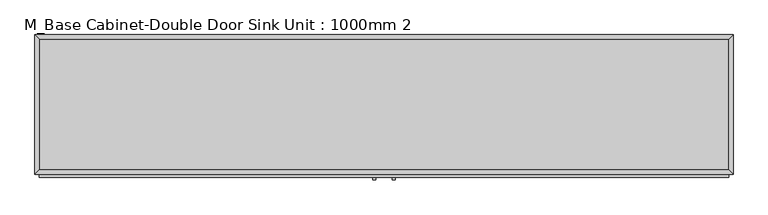
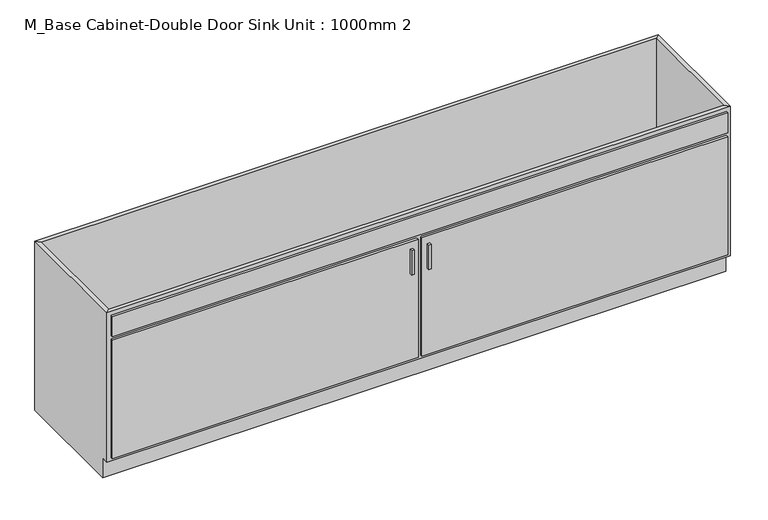
"""IFC4 building model written with IfcOpenShell, lengths in millimetres: furniture geometry, M_Base Cabinet-Double Door Sink Unit : 1000mm 2."""

from ifc_helpers import new_model, si_unit, frame, origin, place, context, project, spatial, polyline, outline, extrude, faceted_brep, source, transform, mapped, element, save


def m_base_cabinet_double_door_sink_unit_1000mm_2_5b8409a6(model_context):
    return source(origin(), model_context, "Body", "SolidModel", [
        faceted_brep([(1499.6877049, -580.95, 860.0), (1499.6877049, -580.95, 100.0), (-1462.2122951, -580.95, 100.0), (-1462.2122951, -580.95, 860.0), (-1481.2622951, -600.0, 860.0), (1518.7377049, -600.0, 860.0), (-1481.2622951, -600.0, 100.0), (1518.7377049, -600.0, 100.0), (-1462.2122951, -565.0, 100.0), (-1462.2122951, -19.05, 100.0), (-1462.2122951, -19.05, 860.0), (-1481.2622951, 0.0, 860.0), (-1481.2622951, 0.0, 0.0), (-1481.2622951, -565.0, 0.0), (-1481.2622951, -565.0, 100.0), (1499.6877049, -19.05, 100.0), (1499.6877049, -19.05, 860.0), (1518.7377049, 0.0, 860.0), (1518.7377049, 0.0, 0.0), (1499.6877049, -565.0, 100.0), (1518.7377049, -565.0, 100.0), (1518.7377049, -565.0, 0.0)], [[[0, 1, 2, 3]], [[0, 3, 4, 5]], [[5, 4, 6, 7]], [[2, 1, 7, 6]], [[3, 2, 8, 9, 10]], [[4, 3, 10, 11]], [[6, 4, 11, 12, 13, 14]], [[2, 6, 14, 8]], [[10, 9, 15, 16]], [[11, 10, 16, 17]], [[12, 11, 17, 18]], [[1, 0, 16, 15, 19]], [[0, 5, 17, 16]], [[5, 7, 20, 21, 18, 17]], [[7, 1, 19, 20]], [[8, 19, 15, 9]], [[18, 21, 13, 12]], [[13, 21, 20, 19, 8, 14]]]),
        extrude(outline(polyline([(-16.1872951, -625.4), (-28.8872951, -625.4), (-28.8872951, -612.7), (-16.1872951, -612.7), (-16.1872951, -625.4)])), frame((0.0, 0.0, 557.469895), z_axis=(0.0, 0.0, 1.0), x_axis=(1.0, 0.0, 0.0)), (0.0, 0.0, 1.0), 124.730105),
        extrude(outline(polyline([(66.3627049, -625.4), (53.6627049, -625.4), (53.6627049, -612.7), (66.3627049, -612.7), (66.3627049, -625.4)])), frame((0.0, 0.0, 557.469895), z_axis=(0.0, 0.0, 1.0), x_axis=(1.0, 0.0, 0.0)), (0.0, 0.0, 1.0), 124.730105),
        extrude(outline(polyline([(9.2127049, -612.7), (-1462.2122951, -612.7), (-1462.2122951, -600.0), (9.2127049, -600.0), (9.2127049, -612.7)])), frame((0.0, 0.0, 119.05), z_axis=(0.0, 0.0, 1.0), x_axis=(1.0, 0.0, 0.0)), (0.0, 0.0, 1.0), 601.25),
        extrude(outline(polyline([(1499.6877049, -612.7), (28.2627049, -612.7), (28.2627049, -600.0), (1499.6877049, -600.0), (1499.6877049, -612.7)])), frame((0.0, 0.0, 119.05), z_axis=(0.0, 0.0, 1.0), x_axis=(1.0, 0.0, 0.0)), (0.0, 0.0, 1.0), 601.25),
        extrude(outline(polyline([(1499.6877049, -612.7), (-1462.2122951, -612.7), (-1462.2122951, -600.0), (1499.6877049, -600.0), (1499.6877049, -612.7)])), frame((0.0, 0.0, 739.35), z_axis=(0.0, 0.0, 1.0), x_axis=(1.0, 0.0, 0.0)), (0.0, 0.0, 1.0), 101.6),
        extrude(outline(polyline([(1499.6877049, -19.05), (1499.6877049, -580.95), (-1462.2122951, -580.95), (-1462.2122951, -19.05), (1499.6877049, -19.05)])), frame((0.0, 0.0, 100.0), z_axis=(0.0, 0.0, 1.0), x_axis=(1.0, 0.0, 0.0)), (0.0, 0.0, 1.0), 19.05),
    ])


if __name__ == "__main__":
    model = new_model("IFC4")
    model_context = context("Model", 3, world=origin())
    ifc_project = project(units=[si_unit("LENGTHUNIT", "METRE", prefix="MILLI")], contexts=[model_context])
    site = spatial("IfcSite", under=ifc_project)
    building = spatial("IfcBuilding", under=site)
    placement = place(None, origin())
    m_base_cabinet_double_door_sink_unit_1000mm_2_shape = m_base_cabinet_double_door_sink_unit_1000mm_2_5b8409a6(model_context)
    element("IfcFurniture", 1, ObjectType="M_Base Cabinet-Double Door Sink Unit : 1000mm 2", at=placement, inside=building, context=model_context, shape_type="MappedRepresentation", body=[
        mapped(m_base_cabinet_double_door_sink_unit_1000mm_2_shape, transform((0.0, 0.0, 0.0), x_axis=(1.0, 0.0, 0.0), y_axis=(0.0, 1.0, 0.0), z_axis=(0.0, 0.0, 1.0))),
    ])
    save(model, "model.ifc")

# Revit data of these elements
# Type "M_Base Cabinet-Double Door Sink Unit : 1000mm 2"
#   Depth = 0.60 m
#   Height = 0.86 m
#   Plinth Depth = 0.035 m
#   Plinth Height = 0.10 m
#   Width = 3.00 m
#   Cabinet Material = none
#   Door/Drawer Material = none
#   Handle Material = Cabinets - Handles
#   Default Elevation = 0
# Element 1 (IfcFurniture, "M_Base Cabinet-Double Door Sink Unit : 1000mm 2")
#   Materials on its faces: "Cabinets", "Cabinets - Handles"
# Materials
#   "Cabinets - Handles": class "Metal", colour RGB 57 57 57, transparency 0
#   "Cabinets": class "Miscellaneous", colour RGB 249 249 249, transparency 0
